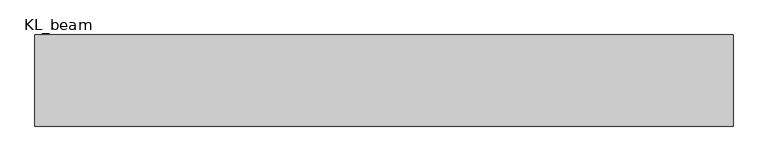
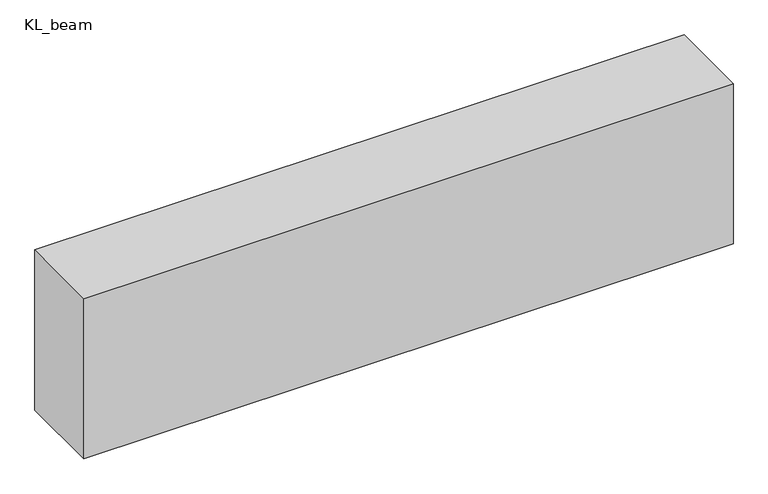
"""IFC4 building model written with IfcOpenShell, lengths in millimetres: beam geometry, 混凝土 - 矩形梁 : KL_beam."""

from ifc_helpers import new_model, si_unit, frame, origin, place, context, project, spatial, polyline, outline, extrude, source, transform, mapped, element, save


def kl_beam_1e568505(model_context):
    return source(origin(), model_context, "Body", "SweptSolid", [
        extrude(outline(polyline([(1532.0, 200.0), (1532.0, -200.0), (-1532.0, -200.0), (-1532.0, 200.0), (1532.0, 200.0)])), frame((0.0, 0.0, -400.0), z_axis=(0.0, 0.0, 1.0), x_axis=(1.0, 0.0, 0.0)), (0.0, 0.0, 1.0), 800.0),
    ])


if __name__ == "__main__":
    model = new_model("IFC4")
    model_context = context("Model", 3, world=origin())
    ifc_project = project(units=[si_unit("LENGTHUNIT", "METRE", prefix="MILLI")], contexts=[model_context])
    site = spatial("IfcSite", under=ifc_project)
    building = spatial("IfcBuilding", under=site)
    placement = place(None, origin())
    kl_beam_shape = kl_beam_1e568505(model_context)
    element("IfcBeam", 1, ObjectType="混凝土 - 矩形梁 : KL_beam", at=placement, inside=building, context=model_context, shape_type="MappedRepresentation", body=[
        mapped(kl_beam_shape, transform((0.0, 0.0, 0.0), x_axis=(1.0, 0.0, 0.0), y_axis=(0.0, 1.0, 0.0), z_axis=(0.0, 0.0, 1.0))),
    ])
    save(model, "model.ifc")

# Revit data of these elements
# Type "混凝土 - 矩形梁 : KL_beam"
#   Length [instance default] = 1524 mm
#   b = 400 mm
#   h = 800 mm
#   Structural Material [instance default] = 混凝土 - 现场浇注混凝土
#   Assembly Code = ""
# Element 1 (IfcBeam, "混凝土 - 矩形梁 : KL_beam")
#   Structural Material = none
# Materials
#   "混凝土 - 现场浇注混凝土": class "混凝土", colour RGB 192 192 192, transparency 0
